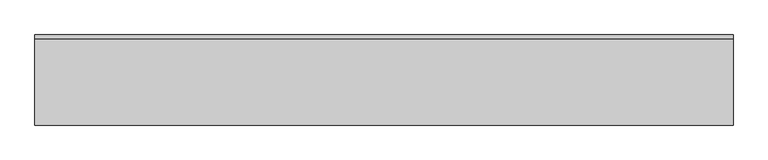
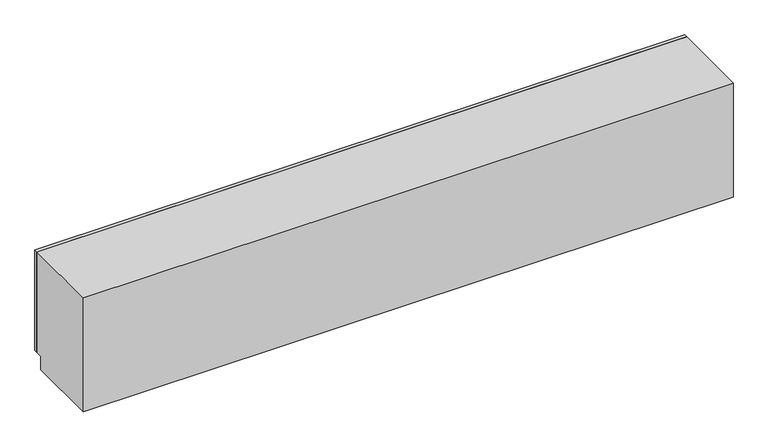
"""IFC4 building model written with IfcOpenShell, lengths in millimetres: furniture geometry, OD_CW_Base Cabinet : OD_CW_Base Cabinet."""

from ifc_helpers import new_model, si_unit, frame, origin, place, context, project, spatial, polyline, outline, extrude, source, transform, mapped, element, save


def furniture_87055c2a(model_context):
    return source(origin(), model_context, "Body", "SweptSolid", [
        extrude(outline(polyline([(18.7377049, -25.4), (18.7377049, 0.0), (4740.5928379, 0.0), (4740.5928379, -25.4), (18.7377049, -25.4)])), frame((0.0, 0.0, 101.6), z_axis=(0.0, 0.0, 1.0), x_axis=(1.0, 0.0, 0.0)), (0.0, 0.0, 1.0), 774.7),
        extrude(outline(polyline([(-25.4, 876.3), (-25.4, 101.6), (-76.2, 101.6), (-76.2, 0.0), (-609.6, 0.0), (-609.6, 876.3), (-25.4, 876.3)])), frame((18.7377049, 0.0, 0.0), z_axis=(1.0, 0.0, 0.0), x_axis=(0.0, 1.0, 0.0)), (0.0, 0.0, 1.0), 4721.855133),
    ])


if __name__ == "__main__":
    model = new_model("IFC4")
    model_context = context("Model", 3, world=origin())
    ifc_project = project(units=[si_unit("LENGTHUNIT", "METRE", prefix="MILLI")], contexts=[model_context])
    site = spatial("IfcSite", under=ifc_project)
    building = spatial("IfcBuilding", under=site)
    placement = place(None, origin())
    furniture_shape = furniture_87055c2a(model_context)
    element("IfcFurniture", 1, ObjectType="OD_CW_Base Cabinet : OD_CW_Base Cabinet", at=placement, inside=building, context=model_context, shape_type="MappedRepresentation", body=[
        mapped(furniture_shape, transform((0.0, 0.0, 0.0), x_axis=(1.0, 0.0, 0.0), y_axis=(0.0, 1.0, 0.0), z_axis=(0.0, 0.0, 1.0))),
    ])
    save(model, "model.ifc")

# Revit data of these elements
# Type "OD_CW_Base Cabinet : OD_CW_Base Cabinet"
#   OD_CW_Width [instance default] = 2' - 10"
#   OD_CW_Length [instance default] = 8' - 0"
#   OD_CW_Height [instance default] = 2' - 3"
#   Depth = 2' - 0"
#   Height = 3' - 0"
#   Width = 4' - 0"
#   OD_CW_Material_Front Panel [instance default] = none
#   OD_CW_Material_Body [instance default] = none
# Element 1 (IfcFurniture, "OD_CW_Base Cabinet : OD_CW_Base Cabinet")
#   OD_CW_Width = 2' - 0"
#   OD_CW_Length = 15' - 5.89981"
#   OD_CW_Height = 2' - 10 1/2"
